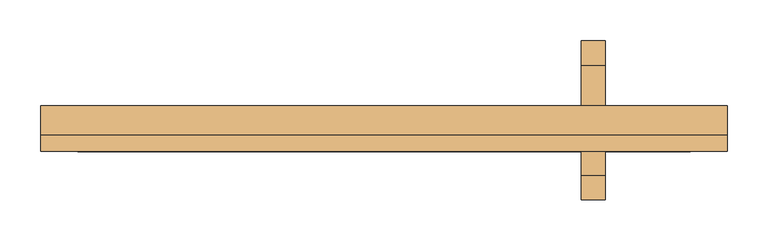
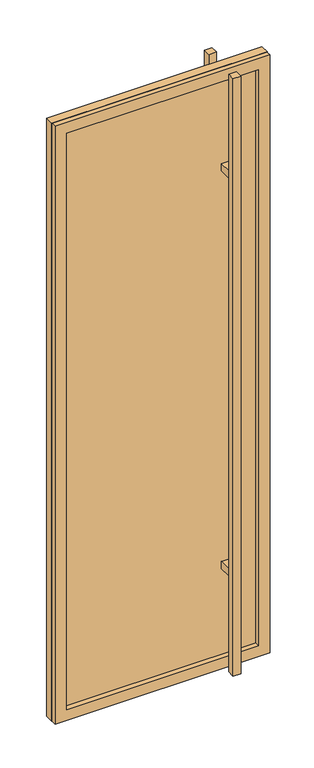
"""IFC4 building model written with IfcOpenShell, lengths in millimetres: door geometry, Anta Singola (1) : Anta Singola (1)."""

import ifcopenshell
import ifcopenshell.guid

model = None  # the IFC model being written
_history = None  # IfcOwnerHistory: only IFC2X3 demands one
_inside = {}  # id of a spatial element -> (the spatial element, [elements in it])
_under = {}  # id of a project, library or spatial element -> (it, [spatial elements below it])
_declared = {}  # id of a project -> (the project, [libraries it declares])
_typed = {}  # id of a type object -> (the type object, [elements of that type])
_made_of = {}  # id of a material, layer set ... -> (it, [elements and type objects made of it])


def new_model(schema):
    """Start an empty IFC model of exactly this schema.

    Asked for "IFC4X3", IfcOpenShell would pick the latest addendum, in which some entities
    have other attributes; the version numbers below select the first issue.
    IFC2X3 requires an IfcOwnerHistory on every rooted entity: one is made here for all.
    """
    global model, _history
    if schema == "IFC4X3":
        model = ifcopenshell.file(schema_version=(4, 3, 0, 0))
    else:
        model = ifcopenshell.file(schema=schema)
    _inside.clear()
    _under.clear()
    _declared.clear()
    _typed.clear()
    _made_of.clear()
    _history = None
    if model.schema == "IFC2X3":
        org = make("IfcOrganization", Name="unknown")
        user = make(
            "IfcPersonAndOrganization",
            ThePerson=make("IfcPerson", FamilyName="unknown"),
            TheOrganization=org,
        )
        app = make(
            "IfcApplication",
            ApplicationDeveloper=org,
            Version="unknown",
            ApplicationFullName="unknown",
            ApplicationIdentifier="unknown",
        )
        _history = make(
            "IfcOwnerHistory",
            OwningUser=user,
            OwningApplication=app,
            ChangeAction="ADDED",
            CreationDate=0,
        )
    return model


def make(cls, **values):
    """One entity of the class cls with the attributes given. An attribute that is None is left unset."""
    return model.create_entity(
        cls, **{name: value for name, value in values.items() if value is not None}
    )


def rooted(cls, **values):
    """An entity with a GlobalId (a new one), such as an element, a storey or a relation."""
    return make(cls, GlobalId=ifcopenshell.guid.new(), OwnerHistory=_history, **values)


def si_unit(unit_type, name, prefix=None):
    """IfcSIUnit, for example si_unit("LENGTHUNIT", "METRE", prefix="MILLI")."""
    return make("IfcSIUnit", UnitType=unit_type, Prefix=prefix, Name=name)


def assignment(units):
    """IfcUnitAssignment: the units of a project."""
    return None if units is None else make("IfcUnitAssignment", Units=units)


def point(xyz):
    """IfcCartesianPoint."""
    return None if xyz is None else make("IfcCartesianPoint", Coordinates=xyz)


def direction(xyz):
    """IfcDirection."""
    return None if xyz is None else make("IfcDirection", DirectionRatios=xyz)


def frame(location, z_axis=None, x_axis=None):
    """IfcAxis2Placement3D, a coordinate frame: its origin and axes. An axis left out is left unset."""
    return make(
        "IfcAxis2Placement3D",
        Location=point(location),
        Axis=direction(z_axis),
        RefDirection=direction(x_axis),
    )


def origin():
    """The frame at (0, 0, 0) with its axes left unset."""
    return frame((0.0, 0.0, 0.0))


def origin_with_axes():
    """The frame at (0, 0, 0) with the z axis (0, 0, 1) and the x axis (1, 0, 0) written out."""
    return frame((0.0, 0.0, 0.0), z_axis=(0.0, 0.0, 1.0), x_axis=(1.0, 0.0, 0.0))


def place(relative_to, where):
    """IfcLocalPlacement: puts the frame where relative to a parent placement (None: the world)."""
    return make(
        "IfcLocalPlacement", PlacementRelTo=relative_to, RelativePlacement=where
    )


def context(
    kind, dimensions, precision=None, world=None, true_north=None, identifier=None
):
    """IfcGeometricRepresentationContext, for example the 3D "Model" context."""
    return make(
        "IfcGeometricRepresentationContext",
        ContextIdentifier=identifier,
        ContextType=kind,
        CoordinateSpaceDimension=dimensions,
        Precision=precision,
        WorldCoordinateSystem=world,
        TrueNorth=true_north,
    )


def project(units=None, contexts=None):
    """IfcProject with its units and contexts."""
    return rooted(
        "IfcProject",
        Name="project",
        RepresentationContexts=contexts,
        UnitsInContext=assignment(units),
    )


def spatial(cls, under=None, at=None, **own):
    """A site, building, storey or space (cls), placed at a placement, below another one or the project."""
    s = rooted(cls, ObjectPlacement=at, **own)
    if under is not None:
        _under.setdefault(under.id(), (under, []))[1].append(s)
    return s


def polyline(points):
    """IfcPolyline through the points."""
    return make("IfcPolyline", Points=[point(p) for p in points])


def outline(outer, holes=None, kind="AREA"):
    """IfcArbitraryClosedProfileDef: a profile drawn as a closed curve; with holes, ...WithVoids."""
    if holes is None:
        return make("IfcArbitraryClosedProfileDef", ProfileType=kind, OuterCurve=outer)
    return make(
        "IfcArbitraryProfileDefWithVoids",
        ProfileType=kind,
        OuterCurve=outer,
        InnerCurves=holes,
    )


def extrude(swept, where, along, depth):
    """IfcExtrudedAreaSolid: the profile swept, set in the frame where, extruded along a direction by depth."""
    return make(
        "IfcExtrudedAreaSolid",
        SweptArea=swept,
        Position=where,
        ExtrudedDirection=direction(along),
        Depth=depth,
    )


def shape(context_of_items, identifier, shape_type, items):
    """IfcShapeRepresentation: the items that make up one representation, for example the "Body"."""
    return make(
        "IfcShapeRepresentation",
        ContextOfItems=context_of_items,
        RepresentationIdentifier=identifier,
        RepresentationType=shape_type,
        Items=items,
    )


def source(mapping_origin, context_of_items, identifier, shape_type, items):
    """IfcRepresentationMap: a shape defined once, which mapped items show again and again."""
    return make(
        "IfcRepresentationMap",
        MappingOrigin=mapping_origin,
        MappedRepresentation=shape(context_of_items, identifier, shape_type, items),
    )


def transform(
    local_origin,
    x_axis=None,
    y_axis=None,
    z_axis=None,
    scale=None,
    scale2=None,
    scale3=None,
    uniform=True,
):
    """IfcCartesianTransformationOperator3D, or its non-uniform kind. x_axis, y_axis, z_axis: its Axis1, 2, 3."""
    if uniform:
        return make(
            "IfcCartesianTransformationOperator3D",
            Axis1=direction(x_axis),
            Axis2=direction(y_axis),
            LocalOrigin=point(local_origin),
            Scale=scale,
            Axis3=direction(z_axis),
        )
    return make(
        "IfcCartesianTransformationOperator3DnonUniform",
        Axis1=direction(x_axis),
        Axis2=direction(y_axis),
        LocalOrigin=point(local_origin),
        Scale=scale,
        Axis3=direction(z_axis),
        Scale2=scale2,
        Scale3=scale3,
    )


def mapped(mapping_source, mapping_target):
    """IfcMappedItem: shows the shape of a source again, moved by a transform."""
    return make(
        "IfcMappedItem", MappingSource=mapping_source, MappingTarget=mapping_target
    )


def made_of(thing, what):
    """Note that an element or type object is made of a material, layer set ...; save() writes the relation."""
    if what is not None:
        _made_of.setdefault(what.id(), (what, []))[1].append(thing)
    return thing


def element(
    cls,
    number,
    at=None,
    inside=None,
    cuts=None,
    type_object=None,
    material=None,
    context=None,
    identifier="Body",
    shape_type=None,
    held_by="IfcProductDefinitionShape",
    body=None,
    shapes=None,
    **own,
):
    """One element of the class cls, such as IfcWall. Its Tag is "e" and its number.

    at: its placement. inside: the storey or other place that contains it. cuts: it is an
    opening in that element (IfcRelVoidsElement). A single representation is given by context,
    identifier, shape_type and body (its items); several are given by shapes. held_by: the class
    of the entity that holds the representations. save() writes the other relations.
    """
    e = rooted(cls, Tag="e%d" % number, ObjectPlacement=at, **own)
    if body is not None:
        shapes = [shape(context, identifier, shape_type, body)]
    if shapes is not None:
        e.Representation = make(held_by, Representations=shapes)
    if inside is not None:
        _inside.setdefault(inside.id(), (inside, []))[1].append(e)
    if cuts is not None:
        rooted(
            "IfcRelVoidsElement", RelatingBuildingElement=cuts, RelatedOpeningElement=e
        )
    if type_object is not None:
        _typed.setdefault(type_object.id(), (type_object, []))[1].append(e)
    return made_of(e, material)


def aggregate(whole, parts):
    """IfcRelAggregates: a whole, such as a stair, and the parts it consists of."""
    return rooted("IfcRelAggregates", RelatingObject=whole, RelatedObjects=parts)


def save(model, path):
    """Write the relations noted so far, then the file.

    IfcRelAggregates (storeys below a building ...), IfcRelContainedInSpatialStructure (elements
    in a storey), IfcRelDefinesByType, IfcRelAssociatesMaterial and IfcRelDeclares: one each for
    every whole, place, type object, material and project.
    """
    for whole, parts in _under.values():
        aggregate(whole, parts)
    for where, things in _inside.values():
        rooted(
            "IfcRelContainedInSpatialStructure",
            RelatedElements=things,
            RelatingStructure=where,
        )
    for kind, things in _typed.values():
        rooted("IfcRelDefinesByType", RelatedObjects=things, RelatingType=kind)
    for what, things in _made_of.values():
        rooted("IfcRelAssociatesMaterial", RelatedObjects=things, RelatingMaterial=what)
    for by, libraries in _declared.values():
        rooted("IfcRelDeclares", RelatingContext=by, RelatedDefinitions=libraries)
    model.write(path)


def door_5ebe6300(model_context):
    return source(origin(), model_context, "Body", "SweptSolid", [
        extrude(outline(polyline([(422.5, -18.0), (-422.5, -18.0), (-422.5, 18.0), (422.5, 18.0), (422.5, -18.0)])), frame((0.0, 0.0, -3.1739529), z_axis=(0.0, 0.0, 1.0), x_axis=(1.0, 0.0, 0.0)), (0.0, 0.0, 1.0), 2478.1739529),
        extrude(outline(polyline([(242.5, -68.0), (272.5, -68.0), (272.5, -98.0), (242.5, -98.0), (242.5, -68.0)])), origin_with_axes(), (0.0, 0.0, 1.0), 2475.0),
        extrude(outline(polyline([(242.5, 98.0), (272.5, 98.0), (272.5, 68.0), (242.5, 68.0), (242.5, 98.0)])), origin_with_axes(), (0.0, 0.0, 1.0), 2475.0),
        extrude(outline(polyline([(2474.5625024, 422.0625024), (2474.5625024, -422.0625024), (-2.7364552, -422.0625024), (-2.7364552, 422.0625024), (2474.5625024, 422.0625024)]), holes=[polyline([(2429.5625024, -377.0625024), (2429.5625024, 377.0625024), (42.2635448, 377.0625024), (42.2635448, -377.0625024), (2429.5625024, -377.0625024)])]), frame((0.0, -38.0, 0.0), z_axis=(0.0, 1.0, 0.0), x_axis=(0.0, 0.0, 1.0)), (0.0, 0.0, 1.0), 20.0),
        extrude(outline(polyline([(272.5, 68.0), (272.5, 18.0), (242.5, 18.0), (242.5, 68.0), (272.5, 68.0)])), frame((0.0, 0.0, 396.8260471), z_axis=(0.0, 0.0, 1.0), x_axis=(1.0, 0.0, 0.0)), (0.0, 0.0, 1.0), 30.0),
        extrude(outline(polyline([(272.5, 68.0), (272.5, 18.0), (242.5, 18.0), (242.5, 68.0), (272.5, 68.0)])), frame((0.0, 0.0, 2045.0), z_axis=(0.0, 0.0, 1.0), x_axis=(1.0, 0.0, 0.0)), (0.0, 0.0, 1.0), 30.0),
        extrude(outline(polyline([(272.5, -18.0), (272.5, -68.0), (242.5, -68.0), (242.5, -18.0), (272.5, -18.0)])), frame((0.0, 0.0, 396.8260471), z_axis=(0.0, 0.0, 1.0), x_axis=(1.0, 0.0, 0.0)), (0.0, 0.0, 1.0), 30.0),
        extrude(outline(polyline([(272.5, -18.0), (272.5, -68.0), (242.5, -68.0), (242.5, -18.0), (272.5, -18.0)])), frame((0.0, 0.0, 2045.0), z_axis=(0.0, 0.0, 1.0), x_axis=(1.0, 0.0, 0.0)), (0.0, 0.0, 1.0), 30.0),
    ])


if __name__ == "__main__":
    model = new_model("IFC4")
    model_context = context("Model", 3, world=origin())
    ifc_project = project(units=[si_unit("LENGTHUNIT", "METRE", prefix="MILLI")], contexts=[model_context])
    site = spatial("IfcSite", under=ifc_project)
    building = spatial("IfcBuilding", under=site)
    placement = place(None, origin())
    door_shape = door_5ebe6300(model_context)
    element("IfcDoor", 1, ObjectType="Anta Singola (1) : Anta Singola (1)", at=placement, inside=building, context=model_context, shape_type="MappedRepresentation", body=[
        mapped(door_shape, transform((0.0, 0.0, 0.0), x_axis=(1.0, 0.0, 0.0), y_axis=(0.0, 1.0, 0.0), z_axis=(0.0, 0.0, 1.0))),
    ])
    save(model, "model.ifc")

# Revit data of these elements
# Type "Anta Singola (1) : Anta Singola (1)"
#   Type Mark = "13"
#   Operation = ""
#   Construction Type = "Scorrimenti"
#   Construction Type Id = "opn-d42"
#   Analytic Construction = "Telaio in metallo con vetro singolo trasparente"
#   Sp = 0.036 m
#   Heat Transfer Coefficient (U) = 6.5580 W/(m²·K)
#   L cornice = 0.045 m
#   Quadro = Default - Vetro
#   Maniglia = none
#   Visual Light Transmittance = 0
#   Solar Heat Gain Coefficient = 0
#   Manufacturer = ""
#   Function = (empty or 0)
# Element 1 (IfcDoor, "Anta Singola (1) : Anta Singola (1)")
#   Materials on its faces: "Maniglia", "Default - Vetro"
# Materials
#   "Default - Vetro": class "Vetro", colour RGB 208 208 208, transparency 0.7, Cost = 0
#   "Maniglia": class "Varie", colour RGB 219 219 219, transparency 0
